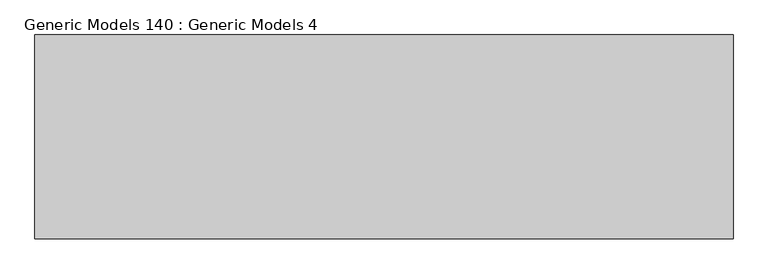
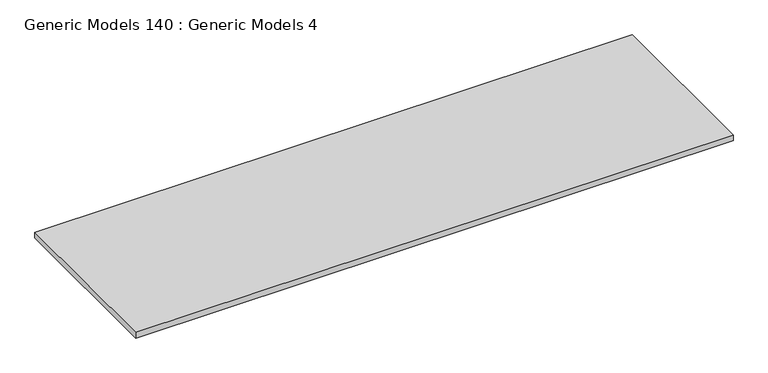
"""IFC4 building model written with IfcOpenShell, lengths in millimetres: proxy geometry, Generic Models 140 : Generic Models 4."""

import ifcopenshell
import ifcopenshell.guid

model = None  # the IFC model being written
_history = None  # IfcOwnerHistory: only IFC2X3 demands one
_inside = {}  # id of a spatial element -> (the spatial element, [elements in it])
_under = {}  # id of a project, library or spatial element -> (it, [spatial elements below it])
_declared = {}  # id of a project -> (the project, [libraries it declares])
_typed = {}  # id of a type object -> (the type object, [elements of that type])
_made_of = {}  # id of a material, layer set ... -> (it, [elements and type objects made of it])


def new_model(schema):
    """Start an empty IFC model of exactly this schema.

    Asked for "IFC4X3", IfcOpenShell would pick the latest addendum, in which some entities
    have other attributes; the version numbers below select the first issue.
    IFC2X3 requires an IfcOwnerHistory on every rooted entity: one is made here for all.
    """
    global model, _history
    if schema == "IFC4X3":
        model = ifcopenshell.file(schema_version=(4, 3, 0, 0))
    else:
        model = ifcopenshell.file(schema=schema)
    _inside.clear()
    _under.clear()
    _declared.clear()
    _typed.clear()
    _made_of.clear()
    _history = None
    if model.schema == "IFC2X3":
        org = make("IfcOrganization", Name="unknown")
        user = make(
            "IfcPersonAndOrganization",
            ThePerson=make("IfcPerson", FamilyName="unknown"),
            TheOrganization=org,
        )
        app = make(
            "IfcApplication",
            ApplicationDeveloper=org,
            Version="unknown",
            ApplicationFullName="unknown",
            ApplicationIdentifier="unknown",
        )
        _history = make(
            "IfcOwnerHistory",
            OwningUser=user,
            OwningApplication=app,
            ChangeAction="ADDED",
            CreationDate=0,
        )
    return model


def make(cls, **values):
    """One entity of the class cls with the attributes given. An attribute that is None is left unset."""
    return model.create_entity(
        cls, **{name: value for name, value in values.items() if value is not None}
    )


def rooted(cls, **values):
    """An entity with a GlobalId (a new one), such as an element, a storey or a relation."""
    return make(cls, GlobalId=ifcopenshell.guid.new(), OwnerHistory=_history, **values)


def si_unit(unit_type, name, prefix=None):
    """IfcSIUnit, for example si_unit("LENGTHUNIT", "METRE", prefix="MILLI")."""
    return make("IfcSIUnit", UnitType=unit_type, Prefix=prefix, Name=name)


def assignment(units):
    """IfcUnitAssignment: the units of a project."""
    return None if units is None else make("IfcUnitAssignment", Units=units)


def point(xyz):
    """IfcCartesianPoint."""
    return None if xyz is None else make("IfcCartesianPoint", Coordinates=xyz)


def direction(xyz):
    """IfcDirection."""
    return None if xyz is None else make("IfcDirection", DirectionRatios=xyz)


def frame(location, z_axis=None, x_axis=None):
    """IfcAxis2Placement3D, a coordinate frame: its origin and axes. An axis left out is left unset."""
    return make(
        "IfcAxis2Placement3D",
        Location=point(location),
        Axis=direction(z_axis),
        RefDirection=direction(x_axis),
    )


def origin():
    """The frame at (0, 0, 0) with its axes left unset."""
    return frame((0.0, 0.0, 0.0))


def place(relative_to, where):
    """IfcLocalPlacement: puts the frame where relative to a parent placement (None: the world)."""
    return make(
        "IfcLocalPlacement", PlacementRelTo=relative_to, RelativePlacement=where
    )


def context(
    kind, dimensions, precision=None, world=None, true_north=None, identifier=None
):
    """IfcGeometricRepresentationContext, for example the 3D "Model" context."""
    return make(
        "IfcGeometricRepresentationContext",
        ContextIdentifier=identifier,
        ContextType=kind,
        CoordinateSpaceDimension=dimensions,
        Precision=precision,
        WorldCoordinateSystem=world,
        TrueNorth=true_north,
    )


def project(units=None, contexts=None):
    """IfcProject with its units and contexts."""
    return rooted(
        "IfcProject",
        Name="project",
        RepresentationContexts=contexts,
        UnitsInContext=assignment(units),
    )


def spatial(cls, under=None, at=None, **own):
    """A site, building, storey or space (cls), placed at a placement, below another one or the project."""
    s = rooted(cls, ObjectPlacement=at, **own)
    if under is not None:
        _under.setdefault(under.id(), (under, []))[1].append(s)
    return s


def polyline(points):
    """IfcPolyline through the points."""
    return make("IfcPolyline", Points=[point(p) for p in points])


def outline(outer, holes=None, kind="AREA"):
    """IfcArbitraryClosedProfileDef: a profile drawn as a closed curve; with holes, ...WithVoids."""
    if holes is None:
        return make("IfcArbitraryClosedProfileDef", ProfileType=kind, OuterCurve=outer)
    return make(
        "IfcArbitraryProfileDefWithVoids",
        ProfileType=kind,
        OuterCurve=outer,
        InnerCurves=holes,
    )


def extrude(swept, where, along, depth):
    """IfcExtrudedAreaSolid: the profile swept, set in the frame where, extruded along a direction by depth."""
    return make(
        "IfcExtrudedAreaSolid",
        SweptArea=swept,
        Position=where,
        ExtrudedDirection=direction(along),
        Depth=depth,
    )


def shape(context_of_items, identifier, shape_type, items):
    """IfcShapeRepresentation: the items that make up one representation, for example the "Body"."""
    return make(
        "IfcShapeRepresentation",
        ContextOfItems=context_of_items,
        RepresentationIdentifier=identifier,
        RepresentationType=shape_type,
        Items=items,
    )


def source(mapping_origin, context_of_items, identifier, shape_type, items):
    """IfcRepresentationMap: a shape defined once, which mapped items show again and again."""
    return make(
        "IfcRepresentationMap",
        MappingOrigin=mapping_origin,
        MappedRepresentation=shape(context_of_items, identifier, shape_type, items),
    )


def transform(
    local_origin,
    x_axis=None,
    y_axis=None,
    z_axis=None,
    scale=None,
    scale2=None,
    scale3=None,
    uniform=True,
):
    """IfcCartesianTransformationOperator3D, or its non-uniform kind. x_axis, y_axis, z_axis: its Axis1, 2, 3."""
    if uniform:
        return make(
            "IfcCartesianTransformationOperator3D",
            Axis1=direction(x_axis),
            Axis2=direction(y_axis),
            LocalOrigin=point(local_origin),
            Scale=scale,
            Axis3=direction(z_axis),
        )
    return make(
        "IfcCartesianTransformationOperator3DnonUniform",
        Axis1=direction(x_axis),
        Axis2=direction(y_axis),
        LocalOrigin=point(local_origin),
        Scale=scale,
        Axis3=direction(z_axis),
        Scale2=scale2,
        Scale3=scale3,
    )


def mapped(mapping_source, mapping_target):
    """IfcMappedItem: shows the shape of a source again, moved by a transform."""
    return make(
        "IfcMappedItem", MappingSource=mapping_source, MappingTarget=mapping_target
    )


def made_of(thing, what):
    """Note that an element or type object is made of a material, layer set ...; save() writes the relation."""
    if what is not None:
        _made_of.setdefault(what.id(), (what, []))[1].append(thing)
    return thing


def element(
    cls,
    number,
    at=None,
    inside=None,
    cuts=None,
    type_object=None,
    material=None,
    context=None,
    identifier="Body",
    shape_type=None,
    held_by="IfcProductDefinitionShape",
    body=None,
    shapes=None,
    **own,
):
    """One element of the class cls, such as IfcWall. Its Tag is "e" and its number.

    at: its placement. inside: the storey or other place that contains it. cuts: it is an
    opening in that element (IfcRelVoidsElement). A single representation is given by context,
    identifier, shape_type and body (its items); several are given by shapes. held_by: the class
    of the entity that holds the representations. save() writes the other relations.
    """
    e = rooted(cls, Tag="e%d" % number, ObjectPlacement=at, **own)
    if body is not None:
        shapes = [shape(context, identifier, shape_type, body)]
    if shapes is not None:
        e.Representation = make(held_by, Representations=shapes)
    if inside is not None:
        _inside.setdefault(inside.id(), (inside, []))[1].append(e)
    if cuts is not None:
        rooted(
            "IfcRelVoidsElement", RelatingBuildingElement=cuts, RelatedOpeningElement=e
        )
    if type_object is not None:
        _typed.setdefault(type_object.id(), (type_object, []))[1].append(e)
    return made_of(e, material)


def aggregate(whole, parts):
    """IfcRelAggregates: a whole, such as a stair, and the parts it consists of."""
    return rooted("IfcRelAggregates", RelatingObject=whole, RelatedObjects=parts)


def save(model, path):
    """Write the relations noted so far, then the file.

    IfcRelAggregates (storeys below a building ...), IfcRelContainedInSpatialStructure (elements
    in a storey), IfcRelDefinesByType, IfcRelAssociatesMaterial and IfcRelDeclares: one each for
    every whole, place, type object, material and project.
    """
    for whole, parts in _under.values():
        aggregate(whole, parts)
    for where, things in _inside.values():
        rooted(
            "IfcRelContainedInSpatialStructure",
            RelatedElements=things,
            RelatingStructure=where,
        )
    for kind, things in _typed.values():
        rooted("IfcRelDefinesByType", RelatedObjects=things, RelatingType=kind)
    for what, things in _made_of.values():
        rooted("IfcRelAssociatesMaterial", RelatedObjects=things, RelatingMaterial=what)
    for by, libraries in _declared.values():
        rooted("IfcRelDeclares", RelatingContext=by, RelatedDefinitions=libraries)
    model.write(path)


def generic_models_140_generic_models_4_f338117d(model_context):
    return source(origin(), model_context, "Body", "SweptSolid", [
        extrude(outline(polyline([(-19489.9914237, 3199.3533277), (-19489.9914237, 6864.6269221), (-6942.3914237, 6864.6269221), (-6942.3914237, 3199.3533277), (-19489.9914237, 3199.3533277)])), frame((0.0, 0.0, 123009.028424), z_axis=(0.0, 0.0, 1.0), x_axis=(1.0, 0.0, 0.0)), (0.0, 0.0, 1.0), 127.0),
    ])


if __name__ == "__main__":
    model = new_model("IFC4")
    model_context = context("Model", 3, world=origin())
    ifc_project = project(units=[si_unit("LENGTHUNIT", "METRE", prefix="MILLI")], contexts=[model_context])
    site = spatial("IfcSite", under=ifc_project)
    building = spatial("IfcBuilding", under=site)
    placement = place(None, origin())
    generic_models_140_generic_models_4_shape = generic_models_140_generic_models_4_f338117d(model_context)
    element("IfcBuildingElementProxy", 1, Name="Generic Models 140 : Generic Models 4", ObjectType="Generic Models 140 : Generic Models 4", at=placement, inside=building, context=model_context, shape_type="MappedRepresentation", body=[
        mapped(generic_models_140_generic_models_4_shape, transform((0.0, 0.0, 0.0), x_axis=(1.0, 0.0, 0.0), y_axis=(0.0, 1.0, 0.0), z_axis=(0.0, 0.0, 1.0))),
    ])
    save(model, "model.ifc")

# Revit data of these elements
# Element 1 (IfcBuildingElementProxy, "Generic Models 140 : Generic Models 4")
#   Materials on its faces: "_CONCRETE SLAB W/ WIRE MESH (SEE STRUCT. DWGS) - SLOPE 1% AWAY FROM BUILDING"
# Materials
#   "_CONCRETE SLAB W/ WIRE MESH (SEE STRUCT. DWGS) - SLOPE 1% AWAY FROM BUILDING": class "Generic", colour RGB 191 191 191, transparency 0, Cost = 0
